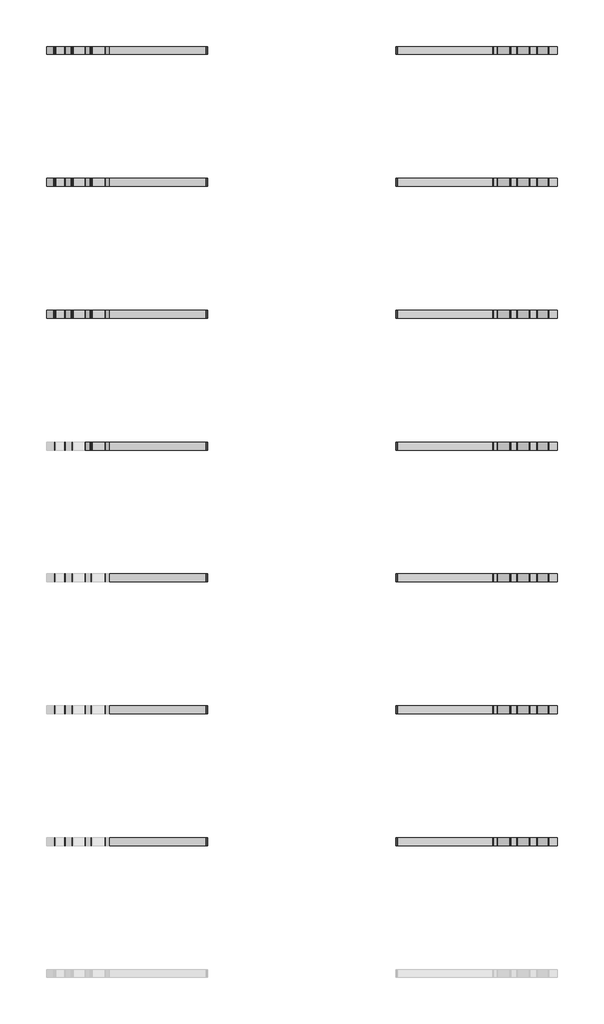
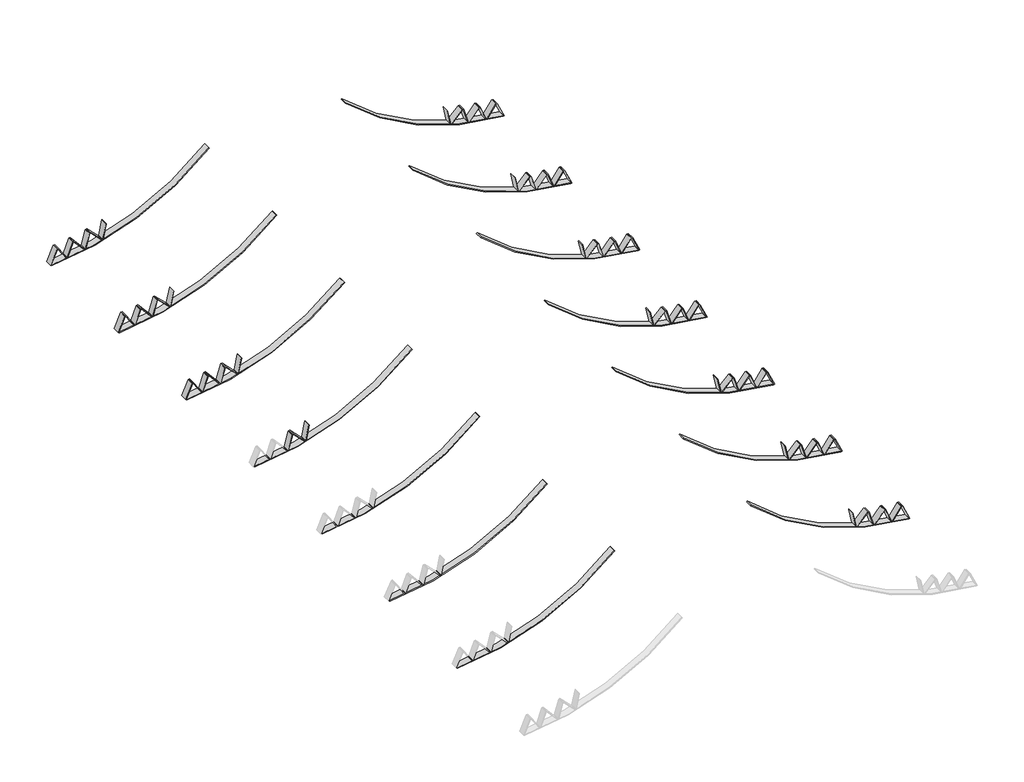
# One storey, part 4 of 4: 87 beams.
"""IFC4 building model written with IfcOpenShell, lengths in millimetres."""

import ifcopenshell
import ifcopenshell.guid

model = None  # the IFC model being written
_history = None  # IfcOwnerHistory: only IFC2X3 demands one
_inside = {}  # id of a spatial element -> (the spatial element, [elements in it])
_under = {}  # id of a project, library or spatial element -> (it, [spatial elements below it])
_declared = {}  # id of a project -> (the project, [libraries it declares])
_typed = {}  # id of a type object -> (the type object, [elements of that type])
_made_of = {}  # id of a material, layer set ... -> (it, [elements and type objects made of it])


def new_model(schema):
    """Start an empty IFC model of exactly this schema.

    Asked for "IFC4X3", IfcOpenShell would pick the latest addendum, in which some entities
    have other attributes; the version numbers below select the first issue.
    IFC2X3 requires an IfcOwnerHistory on every rooted entity: one is made here for all.
    """
    global model, _history
    if schema == "IFC4X3":
        model = ifcopenshell.file(schema_version=(4, 3, 0, 0))
    else:
        model = ifcopenshell.file(schema=schema)
    _inside.clear()
    _under.clear()
    _declared.clear()
    _typed.clear()
    _made_of.clear()
    _history = None
    if model.schema == "IFC2X3":
        org = make("IfcOrganization", Name="unknown")
        user = make(
            "IfcPersonAndOrganization",
            ThePerson=make("IfcPerson", FamilyName="unknown"),
            TheOrganization=org,
        )
        app = make(
            "IfcApplication",
            ApplicationDeveloper=org,
            Version="unknown",
            ApplicationFullName="unknown",
            ApplicationIdentifier="unknown",
        )
        _history = make(
            "IfcOwnerHistory",
            OwningUser=user,
            OwningApplication=app,
            ChangeAction="ADDED",
            CreationDate=0,
        )
    return model


def make(cls, **values):
    """One entity of the class cls with the attributes given. An attribute that is None is left unset."""
    return model.create_entity(
        cls, **{name: value for name, value in values.items() if value is not None}
    )


def rooted(cls, **values):
    """An entity with a GlobalId (a new one), such as an element, a storey or a relation."""
    return make(cls, GlobalId=ifcopenshell.guid.new(), OwnerHistory=_history, **values)


def si_unit(unit_type, name, prefix=None):
    """IfcSIUnit, for example si_unit("LENGTHUNIT", "METRE", prefix="MILLI")."""
    return make("IfcSIUnit", UnitType=unit_type, Prefix=prefix, Name=name)


def assignment(units):
    """IfcUnitAssignment: the units of a project."""
    return None if units is None else make("IfcUnitAssignment", Units=units)


def point(xyz):
    """IfcCartesianPoint."""
    return None if xyz is None else make("IfcCartesianPoint", Coordinates=xyz)


def direction(xyz):
    """IfcDirection."""
    return None if xyz is None else make("IfcDirection", DirectionRatios=xyz)


def frame(location, z_axis=None, x_axis=None):
    """IfcAxis2Placement3D, a coordinate frame: its origin and axes. An axis left out is left unset."""
    return make(
        "IfcAxis2Placement3D",
        Location=point(location),
        Axis=direction(z_axis),
        RefDirection=direction(x_axis),
    )


def frame_2d(location, x_axis=None):
    """IfcAxis2Placement2D, a coordinate frame in the plane: its origin and x axis."""
    return make(
        "IfcAxis2Placement2D", Location=point(location), RefDirection=direction(x_axis)
    )


def origin():
    """The frame at (0, 0, 0) with its axes left unset."""
    return frame((0.0, 0.0, 0.0))


def place(relative_to, where):
    """IfcLocalPlacement: puts the frame where relative to a parent placement (None: the world)."""
    return make(
        "IfcLocalPlacement", PlacementRelTo=relative_to, RelativePlacement=where
    )


def context(
    kind, dimensions, precision=None, world=None, true_north=None, identifier=None
):
    """IfcGeometricRepresentationContext, for example the 3D "Model" context."""
    return make(
        "IfcGeometricRepresentationContext",
        ContextIdentifier=identifier,
        ContextType=kind,
        CoordinateSpaceDimension=dimensions,
        Precision=precision,
        WorldCoordinateSystem=world,
        TrueNorth=true_north,
    )


def project(units=None, contexts=None):
    """IfcProject with its units and contexts."""
    return rooted(
        "IfcProject",
        Name="project",
        RepresentationContexts=contexts,
        UnitsInContext=assignment(units),
    )


def spatial(cls, under=None, at=None, **own):
    """A site, building, storey or space (cls), placed at a placement, below another one or the project."""
    s = rooted(cls, ObjectPlacement=at, **own)
    if under is not None:
        _under.setdefault(under.id(), (under, []))[1].append(s)
    return s


def polyline(points):
    """IfcPolyline through the points."""
    return make("IfcPolyline", Points=[point(p) for p in points])


def circle_curve(where, radius):
    """IfcCircle in the frame where."""
    return make("IfcCircle", Position=where, Radius=radius)


def trimmed(basis, trim1, trim2, sense, master):
    """IfcTrimmedCurve: the piece of a basis curve between two trims."""
    return make(
        "IfcTrimmedCurve",
        BasisCurve=basis,
        Trim1=trim1,
        Trim2=trim2,
        SenseAgreement=sense,
        MasterRepresentation=master,
    )


def segment(curve, same_sense, transition):
    """IfcCompositeCurveSegment."""
    return make(
        "IfcCompositeCurveSegment",
        Transition=transition,
        SameSense=same_sense,
        ParentCurve=curve,
    )


def composite_curve(segments, self_intersect=None):
    """IfcCompositeCurve: segments joined end to end."""
    return make("IfcCompositeCurve", Segments=segments, SelfIntersect=self_intersect)


def outline(outer, holes=None, kind="AREA"):
    """IfcArbitraryClosedProfileDef: a profile drawn as a closed curve; with holes, ...WithVoids."""
    if holes is None:
        return make("IfcArbitraryClosedProfileDef", ProfileType=kind, OuterCurve=outer)
    return make(
        "IfcArbitraryProfileDefWithVoids",
        ProfileType=kind,
        OuterCurve=outer,
        InnerCurves=holes,
    )


def extrude(swept, where, along, depth):
    """IfcExtrudedAreaSolid: the profile swept, set in the frame where, extruded along a direction by depth."""
    return make(
        "IfcExtrudedAreaSolid",
        SweptArea=swept,
        Position=where,
        ExtrudedDirection=direction(along),
        Depth=depth,
    )


def shape(context_of_items, identifier, shape_type, items):
    """IfcShapeRepresentation: the items that make up one representation, for example the "Body"."""
    return make(
        "IfcShapeRepresentation",
        ContextOfItems=context_of_items,
        RepresentationIdentifier=identifier,
        RepresentationType=shape_type,
        Items=items,
    )


def source(mapping_origin, context_of_items, identifier, shape_type, items):
    """IfcRepresentationMap: a shape defined once, which mapped items show again and again."""
    return make(
        "IfcRepresentationMap",
        MappingOrigin=mapping_origin,
        MappedRepresentation=shape(context_of_items, identifier, shape_type, items),
    )


def transform(
    local_origin,
    x_axis=None,
    y_axis=None,
    z_axis=None,
    scale=None,
    scale2=None,
    scale3=None,
    uniform=True,
):
    """IfcCartesianTransformationOperator3D, or its non-uniform kind. x_axis, y_axis, z_axis: its Axis1, 2, 3."""
    if uniform:
        return make(
            "IfcCartesianTransformationOperator3D",
            Axis1=direction(x_axis),
            Axis2=direction(y_axis),
            LocalOrigin=point(local_origin),
            Scale=scale,
            Axis3=direction(z_axis),
        )
    return make(
        "IfcCartesianTransformationOperator3DnonUniform",
        Axis1=direction(x_axis),
        Axis2=direction(y_axis),
        LocalOrigin=point(local_origin),
        Scale=scale,
        Axis3=direction(z_axis),
        Scale2=scale2,
        Scale3=scale3,
    )


def mapped(mapping_source, mapping_target):
    """IfcMappedItem: shows the shape of a source again, moved by a transform."""
    return make(
        "IfcMappedItem", MappingSource=mapping_source, MappingTarget=mapping_target
    )


def made_of(thing, what):
    """Note that an element or type object is made of a material, layer set ...; save() writes the relation."""
    if what is not None:
        _made_of.setdefault(what.id(), (what, []))[1].append(thing)
    return thing


def element(
    cls,
    number,
    at=None,
    inside=None,
    cuts=None,
    type_object=None,
    material=None,
    context=None,
    identifier="Body",
    shape_type=None,
    held_by="IfcProductDefinitionShape",
    body=None,
    shapes=None,
    **own,
):
    """One element of the class cls, such as IfcWall. Its Tag is "e" and its number.

    at: its placement. inside: the storey or other place that contains it. cuts: it is an
    opening in that element (IfcRelVoidsElement). A single representation is given by context,
    identifier, shape_type and body (its items); several are given by shapes. held_by: the class
    of the entity that holds the representations. save() writes the other relations.
    """
    e = rooted(cls, Tag="e%d" % number, ObjectPlacement=at, **own)
    if body is not None:
        shapes = [shape(context, identifier, shape_type, body)]
    if shapes is not None:
        e.Representation = make(held_by, Representations=shapes)
    if inside is not None:
        _inside.setdefault(inside.id(), (inside, []))[1].append(e)
    if cuts is not None:
        rooted(
            "IfcRelVoidsElement", RelatingBuildingElement=cuts, RelatedOpeningElement=e
        )
    if type_object is not None:
        _typed.setdefault(type_object.id(), (type_object, []))[1].append(e)
    return made_of(e, material)


def aggregate(whole, parts):
    """IfcRelAggregates: a whole, such as a stair, and the parts it consists of."""
    return rooted("IfcRelAggregates", RelatingObject=whole, RelatedObjects=parts)


def save(model, path):
    """Write the relations noted so far, then the file.

    IfcRelAggregates (storeys below a building ...), IfcRelContainedInSpatialStructure (elements
    in a storey), IfcRelDefinesByType, IfcRelAssociatesMaterial and IfcRelDeclares: one each for
    every whole, place, type object, material and project.
    """
    for whole, parts in _under.values():
        aggregate(whole, parts)
    for where, things in _inside.values():
        rooted(
            "IfcRelContainedInSpatialStructure",
            RelatedElements=things,
            RelatingStructure=where,
        )
    for kind, things in _typed.values():
        rooted("IfcRelDefinesByType", RelatedObjects=things, RelatingType=kind)
    for what, things in _made_of.values():
        rooted("IfcRelAssociatesMaterial", RelatedObjects=things, RelatingMaterial=what)
    for by, libraries in _declared.values():
        rooted("IfcRelDeclares", RelatingContext=by, RelatedDefinitions=libraries)
    model.write(path)


def placa_diagonal_a71479e9(model_context):
    return source(origin(), model_context, "Body", "SweptSolid", [
        extrude(outline(polyline([(161.178496, 75.0), (161.178496, -75.0), (-185.3041805, -75.0), (-185.3041805, 75.0), (161.178496, 75.0)])), frame((0.0, 0.0, -4.0), z_axis=(0.0, 0.0, 1.0), x_axis=(1.0, 0.0, 0.0)), (0.0, 0.0, 1.0), 8.0),
    ])


def placa_diagonal_67ce8334(model_context):
    return source(origin(), model_context, "Body", "SweptSolid", [
        extrude(outline(polyline([(162.9623469, 75.0), (162.9623469, -75.0), (-162.6761246, -75.0), (-162.6761246, 75.0), (162.9623469, 75.0)])), frame((0.0, 0.0, -4.0), z_axis=(0.0, 0.0, 1.0), x_axis=(1.0, 0.0, 0.0)), (0.0, 0.0, 1.0), 8.0),
    ])


def placa_diagonal_af2a04a3(model_context):
    return source(origin(), model_context, "Body", "SweptSolid", [
        extrude(outline(polyline([(165.1705216, 75.0), (165.1705216, -75.0), (-165.4962729, -75.0), (-165.4962729, 75.0), (165.1705216, 75.0)])), frame((0.0, 0.0, -4.0), z_axis=(0.0, 0.0, 1.0), x_axis=(1.0, 0.0, 0.0)), (0.0, 0.0, 1.0), 8.0),
    ])


def placa_diagonal_fb53ba7d(model_context):
    return source(origin(), model_context, "Body", "SweptSolid", [
        extrude(outline(polyline([(169.971959, 75.0), (169.971959, -75.0), (-169.5739242, -75.0), (-169.5739242, 75.0), (169.971959, 75.0)])), frame((0.0, 0.0, -4.0), z_axis=(0.0, 0.0, 1.0), x_axis=(1.0, 0.0, 0.0)), (0.0, 0.0, 1.0), 8.0),
    ])


def placa_diagonal_d1da0e1c(model_context):
    return source(origin(), model_context, "Body", "SweptSolid", [
        extrude(outline(polyline([(165.1705221, 75.0), (165.1705221, -75.0), (-165.4962734, -75.0), (-165.4962734, 75.0), (165.1705221, 75.0)])), frame((0.0, 0.0, -4.0), z_axis=(0.0, 0.0, 1.0), x_axis=(1.0, 0.0, 0.0)), (0.0, 0.0, 1.0), 8.0),
    ])


def placa_diagonal_6d03bdc5(model_context):
    return source(origin(), model_context, "Body", "SweptSolid", [
        extrude(outline(polyline([(191.209825, 75.0), (191.209825, -75.0), (-166.9394885, -75.0), (-166.9394885, 75.0), (191.209825, 75.0)])), frame((0.0, 0.0, -4.0), z_axis=(0.0, 0.0, 1.0), x_axis=(1.0, 0.0, 0.0)), (0.0, 0.0, 1.0), 8.0),
    ])


def placa_diagonal_30fa4039(model_context):
    return source(origin(), model_context, "Body", "SweptSolid", [
        extrude(outline(polyline([(167.0675386, 75.0), (167.0675386, -75.0), (-167.4240159, -75.0), (-167.4240159, 75.0), (167.0675386, 75.0)])), frame((0.0, 0.0, -4.0), z_axis=(0.0, 0.0, 1.0), x_axis=(1.0, 0.0, 0.0)), (0.0, 0.0, 1.0), 8.0),
    ])


def placa_diagonal_ded414cc(model_context):
    return source(origin(), model_context, "Body", "SweptSolid", [
        extrude(outline(polyline([(167.4240165, 75.0), (167.4240165, -75.0), (-167.0675392, -75.0), (-167.0675392, 75.0), (167.4240165, 75.0)])), frame((0.0, 0.0, -4.0), z_axis=(0.0, 0.0, 1.0), x_axis=(1.0, 0.0, 0.0)), (0.0, 0.0, 1.0), 8.0),
    ])


def placa_diagonal_4690b74a(model_context):
    return source(origin(), model_context, "Body", "SweptSolid", [
        extrude(outline(polyline([(167.0675389, 75.0), (167.0675389, -75.0), (-167.4240162, -75.0), (-167.4240162, 75.0), (167.0675389, 75.0)])), frame((0.0, 0.0, -4.0), z_axis=(0.0, 0.0, 1.0), x_axis=(1.0, 0.0, 0.0)), (0.0, 0.0, 1.0), 8.0),
    ])


def placa_diagonal_aaf0c3b6(model_context):
    return source(origin(), model_context, "Body", "SweptSolid", [
        extrude(outline(polyline([(167.4240163, 75.0), (167.4240163, -75.0), (-167.067539, -75.0), (-167.067539, 75.0), (167.4240163, 75.0)])), frame((0.0, 0.0, -4.0), z_axis=(0.0, 0.0, 1.0), x_axis=(1.0, 0.0, 0.0)), (0.0, 0.0, 1.0), 8.0),
    ])


model = new_model("IFC4")

# Units and contexts
model_context = context("Model", 3, world=origin())
ifc_project = project(units=[si_unit("LENGTHUNIT", "METRE", prefix="MILLI")], contexts=[model_context])

# Site, building, storey
site = spatial("IfcSite", under=ifc_project)
building = spatial("IfcBuilding", under=site)
storey = spatial("IfcBuildingStorey", under=building, Name="Nível 4", Elevation=48165.0)

# Beams
placement = place(None, origin())
element("IfcBeam", 1, ObjectType="Placa : banzo", at=placement, inside=storey, context=model_context, shape_type="SweptSolid", body=[
    extrude(outline(composite_curve([segment(polyline([(48158.5516223, 8114.9704041), (48174.5198715, 8115.9778843)]), True, "CONTINUOUS"), segment(trimmed(circle_curve(frame_2d((53506.1312788, 8452.3636953)), 5342.2126139), [point((48174.5198715, 8115.9778843))], [point((49646.1683419, 4759.1372282))], True, "CARTESIAN"), True, "CONTINUOUS"), segment(polyline([(49646.1683419, 4759.1372282), (49634.6077, 4748.0759643)]), True, "CONTINUOUS"), segment(trimmed(circle_curve(frame_2d((53506.1312788, 8452.3636953)), 5358.2126139), [point((49634.6077, 4748.0759643))], [point((48158.5516223, 8114.9704041))], False, "CARTESIAN"), True, "CONTINUOUS")], self_intersect=False)), frame((0.0, 15321.4376366, 0.0), z_axis=(0.0, 1.0, 0.0), x_axis=(0.0, 0.0, 1.0)), (0.0, 0.0, 1.0), 150.0),
])
element("IfcBeam", 2, ObjectType="Placa : banzo", at=placement, inside=storey, context=model_context, shape_type="SweptSolid", body=[
    extrude(outline(composite_curve([segment(polyline([(49634.6077, 1843.8240278), (49646.1683419, 1832.762764)]), True, "CONTINUOUS"), segment(trimmed(circle_curve(frame_2d((53506.1312788, -1860.4637031)), 5342.2126139), [point((49646.1683419, 1832.762764))], [point((48174.5198715, -1524.0778921))], True, "CARTESIAN"), True, "CONTINUOUS"), segment(polyline([(48174.5198715, -1524.0778921), (48158.5516223, -1523.070412)]), True, "CONTINUOUS"), segment(trimmed(circle_curve(frame_2d((53506.1312788, -1860.4637031)), 5358.2126139), [point((48158.5516223, -1523.070412))], [point((49634.6077, 1843.8240278))], False, "CARTESIAN"), True, "CONTINUOUS")], self_intersect=False)), frame((0.0, 15321.4376366, 0.0), z_axis=(0.0, 1.0, 0.0), x_axis=(0.0, 0.0, 1.0)), (0.0, 0.0, 1.0), 150.0),
])
element("IfcBeam", 3, ObjectType="Placa : banzo", at=placement, inside=storey, context=model_context, shape_type="SweptSolid", body=[
    extrude(outline(composite_curve([segment(polyline([(48158.5516223, 8114.9704041), (48174.5198715, 8115.9778843)]), True, "CONTINUOUS"), segment(trimmed(circle_curve(frame_2d((53506.1312788, 8452.3636953)), 5342.2126139), [point((48174.5198715, 8115.9778843))], [point((49646.1683419, 4759.1372282))], True, "CARTESIAN"), True, "CONTINUOUS"), segment(polyline([(49646.1683419, 4759.1372282), (49634.6077, 4748.0759643)]), True, "CONTINUOUS"), segment(trimmed(circle_curve(frame_2d((53506.1312788, 8452.3636953)), 5358.2126139), [point((49634.6077, 4748.0759643))], [point((48158.5516223, 8114.9704041))], False, "CARTESIAN"), True, "CONTINUOUS")], self_intersect=False)), frame((0.0, 12821.4376366, 0.0), z_axis=(0.0, 1.0, 0.0), x_axis=(0.0, 0.0, 1.0)), (0.0, 0.0, 1.0), 150.0),
])
element("IfcBeam", 4, ObjectType="Placa : banzo", at=placement, inside=storey, context=model_context, shape_type="SweptSolid", body=[
    extrude(outline(composite_curve([segment(polyline([(49634.6077, 1843.8240278), (49646.1683419, 1832.762764)]), True, "CONTINUOUS"), segment(trimmed(circle_curve(frame_2d((53506.1312788, -1860.4637031)), 5342.2126139), [point((49646.1683419, 1832.762764))], [point((48174.5198715, -1524.0778921))], True, "CARTESIAN"), True, "CONTINUOUS"), segment(polyline([(48174.5198715, -1524.0778921), (48158.5516223, -1523.070412)]), True, "CONTINUOUS"), segment(trimmed(circle_curve(frame_2d((53506.1312788, -1860.4637031)), 5358.2126139), [point((48158.5516223, -1523.070412))], [point((49634.6077, 1843.8240278))], False, "CARTESIAN"), True, "CONTINUOUS")], self_intersect=False)), frame((0.0, 12821.4376366, 0.0), z_axis=(0.0, 1.0, 0.0), x_axis=(0.0, 0.0, 1.0)), (0.0, 0.0, 1.0), 150.0),
])
element("IfcBeam", 5, ObjectType="Placa : banzo", at=placement, inside=storey, context=model_context, shape_type="SweptSolid", body=[
    extrude(outline(composite_curve([segment(polyline([(48158.5516223, 8114.9704041), (48174.5198715, 8115.9778843)]), True, "CONTINUOUS"), segment(trimmed(circle_curve(frame_2d((53506.1312788, 8452.3636953)), 5342.2126139), [point((48174.5198715, 8115.9778843))], [point((49646.1683419, 4759.1372282))], True, "CARTESIAN"), True, "CONTINUOUS"), segment(polyline([(49646.1683419, 4759.1372282), (49634.6077, 4748.0759643)]), True, "CONTINUOUS"), segment(trimmed(circle_curve(frame_2d((53506.1312788, 8452.3636953)), 5358.2126139), [point((49634.6077, 4748.0759643))], [point((48158.5516223, 8114.9704041))], False, "CARTESIAN"), True, "CONTINUOUS")], self_intersect=False)), frame((0.0, 10321.4376366, 0.0), z_axis=(0.0, 1.0, 0.0), x_axis=(0.0, 0.0, 1.0)), (0.0, 0.0, 1.0), 150.0),
])
element("IfcBeam", 6, ObjectType="Placa : banzo", at=placement, inside=storey, context=model_context, shape_type="SweptSolid", body=[
    extrude(outline(composite_curve([segment(polyline([(49634.6077, 1843.8240278), (49646.1683419, 1832.762764)]), True, "CONTINUOUS"), segment(trimmed(circle_curve(frame_2d((53506.1312788, -1860.4637031)), 5342.2126139), [point((49646.1683419, 1832.762764))], [point((48174.5198715, -1524.0778921))], True, "CARTESIAN"), True, "CONTINUOUS"), segment(polyline([(48174.5198715, -1524.0778921), (48158.5516223, -1523.070412)]), True, "CONTINUOUS"), segment(trimmed(circle_curve(frame_2d((53506.1312788, -1860.4637031)), 5358.2126139), [point((48158.5516223, -1523.070412))], [point((49634.6077, 1843.8240278))], False, "CARTESIAN"), True, "CONTINUOUS")], self_intersect=False)), frame((0.0, 10321.4376366, 0.0), z_axis=(0.0, 1.0, 0.0), x_axis=(0.0, 0.0, 1.0)), (0.0, 0.0, 1.0), 150.0),
])
element("IfcBeam", 7, ObjectType="Placa : banzo", at=placement, inside=storey, context=model_context, shape_type="SweptSolid", body=[
    extrude(outline(composite_curve([segment(polyline([(48158.5516223, 8114.9704041), (48174.5198715, 8115.9778843)]), True, "CONTINUOUS"), segment(trimmed(circle_curve(frame_2d((53506.1312788, 8452.3636953)), 5342.2126139), [point((48174.5198715, 8115.9778843))], [point((49646.1683419, 4759.1372282))], True, "CARTESIAN"), True, "CONTINUOUS"), segment(polyline([(49646.1683419, 4759.1372282), (49634.6077, 4748.0759643)]), True, "CONTINUOUS"), segment(trimmed(circle_curve(frame_2d((53506.1312788, 8452.3636953)), 5358.2126139), [point((49634.6077, 4748.0759643))], [point((48158.5516223, 8114.9704041))], False, "CARTESIAN"), True, "CONTINUOUS")], self_intersect=False)), frame((0.0, 7821.4376366, 0.0), z_axis=(0.0, 1.0, 0.0), x_axis=(0.0, 0.0, 1.0)), (0.0, 0.0, 1.0), 150.0),
])
element("IfcBeam", 8, ObjectType="Placa : banzo", at=placement, inside=storey, context=model_context, shape_type="SweptSolid", body=[
    extrude(outline(composite_curve([segment(polyline([(49634.6077, 1843.8240278), (49646.1683419, 1832.762764)]), True, "CONTINUOUS"), segment(trimmed(circle_curve(frame_2d((53506.1312788, -1860.4637031)), 5342.2126139), [point((49646.1683419, 1832.762764))], [point((48174.5198715, -1524.0778921))], True, "CARTESIAN"), True, "CONTINUOUS"), segment(polyline([(48174.5198715, -1524.0778921), (48158.5516223, -1523.070412)]), True, "CONTINUOUS"), segment(trimmed(circle_curve(frame_2d((53506.1312788, -1860.4637031)), 5358.2126139), [point((48158.5516223, -1523.070412))], [point((49634.6077, 1843.8240278))], False, "CARTESIAN"), True, "CONTINUOUS")], self_intersect=False)), frame((0.0, 7821.4376366, 0.0), z_axis=(0.0, 1.0, 0.0), x_axis=(0.0, 0.0, 1.0)), (0.0, 0.0, 1.0), 150.0),
])
element("IfcBeam", 9, ObjectType="Placa : banzo", at=placement, inside=storey, context=model_context, shape_type="SweptSolid", body=[
    extrude(outline(composite_curve([segment(polyline([(48158.5516223, 8114.9704041), (48174.5198715, 8115.9778843)]), True, "CONTINUOUS"), segment(trimmed(circle_curve(frame_2d((53506.1312788, 8452.3636953)), 5342.2126139), [point((48174.5198715, 8115.9778843))], [point((49646.1683419, 4759.1372282))], True, "CARTESIAN"), True, "CONTINUOUS"), segment(polyline([(49646.1683419, 4759.1372282), (49634.6077, 4748.0759643)]), True, "CONTINUOUS"), segment(trimmed(circle_curve(frame_2d((53506.1312788, 8452.3636953)), 5358.2126139), [point((49634.6077, 4748.0759643))], [point((48158.5516223, 8114.9704041))], False, "CARTESIAN"), True, "CONTINUOUS")], self_intersect=False)), frame((0.0, 5321.4376366, 0.0), z_axis=(0.0, 1.0, 0.0), x_axis=(0.0, 0.0, 1.0)), (0.0, 0.0, 1.0), 150.0),
])
element("IfcBeam", 10, ObjectType="Placa : banzo", at=placement, inside=storey, context=model_context, shape_type="SweptSolid", body=[
    extrude(outline(composite_curve([segment(polyline([(49634.6077, 1843.8240278), (49646.1683419, 1832.762764)]), True, "CONTINUOUS"), segment(trimmed(circle_curve(frame_2d((53506.1312788, -1860.4637031)), 5342.2126139), [point((49646.1683419, 1832.762764))], [point((48174.5198715, -1524.0778921))], True, "CARTESIAN"), True, "CONTINUOUS"), segment(polyline([(48174.5198715, -1524.0778921), (48158.5516223, -1523.070412)]), True, "CONTINUOUS"), segment(trimmed(circle_curve(frame_2d((53506.1312788, -1860.4637031)), 5358.2126139), [point((48158.5516223, -1523.070412))], [point((49634.6077, 1843.8240278))], False, "CARTESIAN"), True, "CONTINUOUS")], self_intersect=False)), frame((0.0, 5321.4376366, 0.0), z_axis=(0.0, 1.0, 0.0), x_axis=(0.0, 0.0, 1.0)), (0.0, 0.0, 1.0), 150.0),
])
element("IfcBeam", 11, ObjectType="Placa : banzo", at=placement, inside=storey, context=model_context, shape_type="SweptSolid", body=[
    extrude(outline(composite_curve([segment(polyline([(48158.5516223, 8114.9704041), (48174.5198715, 8115.9778843)]), True, "CONTINUOUS"), segment(trimmed(circle_curve(frame_2d((53506.1312788, 8452.3636953)), 5342.2126139), [point((48174.5198715, 8115.9778843))], [point((49646.1683419, 4759.1372282))], True, "CARTESIAN"), True, "CONTINUOUS"), segment(polyline([(49646.1683419, 4759.1372282), (49634.6077, 4748.0759643)]), True, "CONTINUOUS"), segment(trimmed(circle_curve(frame_2d((53506.1312788, 8452.3636953)), 5358.2126139), [point((49634.6077, 4748.0759643))], [point((48158.5516223, 8114.9704041))], False, "CARTESIAN"), True, "CONTINUOUS")], self_intersect=False)), frame((0.0, 2821.4376366, 0.0), z_axis=(0.0, 1.0, 0.0), x_axis=(0.0, 0.0, 1.0)), (0.0, 0.0, 1.0), 150.0),
])
element("IfcBeam", 12, ObjectType="Placa : banzo", at=placement, inside=storey, context=model_context, shape_type="SweptSolid", body=[
    extrude(outline(composite_curve([segment(polyline([(49634.6077, 1843.8240278), (49646.1683419, 1832.762764)]), True, "CONTINUOUS"), segment(trimmed(circle_curve(frame_2d((53506.1312788, -1860.4637031)), 5342.2126139), [point((49646.1683419, 1832.762764))], [point((48174.5198715, -1524.0778921))], True, "CARTESIAN"), True, "CONTINUOUS"), segment(polyline([(48174.5198715, -1524.0778921), (48158.5516223, -1523.070412)]), True, "CONTINUOUS"), segment(trimmed(circle_curve(frame_2d((53506.1312788, -1860.4637031)), 5358.2126139), [point((48158.5516223, -1523.070412))], [point((49634.6077, 1843.8240278))], False, "CARTESIAN"), True, "CONTINUOUS")], self_intersect=False)), frame((0.0, 2821.4376366, 0.0), z_axis=(0.0, 1.0, 0.0), x_axis=(0.0, 0.0, 1.0)), (0.0, 0.0, 1.0), 150.0),
])
element("IfcBeam", 13, ObjectType="Placa : banzo", at=placement, inside=storey, context=model_context, shape_type="SweptSolid", body=[
    extrude(outline(composite_curve([segment(polyline([(48158.5516223, 8114.9704041), (48174.5198715, 8115.9778843)]), True, "CONTINUOUS"), segment(trimmed(circle_curve(frame_2d((53506.1312788, 8452.3636953)), 5342.2126139), [point((48174.5198715, 8115.9778843))], [point((49646.1683419, 4759.1372282))], True, "CARTESIAN"), True, "CONTINUOUS"), segment(polyline([(49646.1683419, 4759.1372282), (49634.6077, 4748.0759643)]), True, "CONTINUOUS"), segment(trimmed(circle_curve(frame_2d((53506.1312788, 8452.3636953)), 5358.2126139), [point((49634.6077, 4748.0759643))], [point((48158.5516223, 8114.9704041))], False, "CARTESIAN"), True, "CONTINUOUS")], self_intersect=False)), frame((0.0, 321.4376366, 0.0), z_axis=(0.0, 1.0, 0.0), x_axis=(0.0, 0.0, 1.0)), (0.0, 0.0, 1.0), 150.0),
])
element("IfcBeam", 14, ObjectType="Placa : banzo", at=placement, inside=storey, context=model_context, shape_type="SweptSolid", body=[
    extrude(outline(composite_curve([segment(polyline([(49634.6077, 1843.8240278), (49646.1683419, 1832.762764)]), True, "CONTINUOUS"), segment(trimmed(circle_curve(frame_2d((53506.1312788, -1860.4637031)), 5342.2126139), [point((49646.1683419, 1832.762764))], [point((48174.5198715, -1524.0778921))], True, "CARTESIAN"), True, "CONTINUOUS"), segment(polyline([(48174.5198715, -1524.0778921), (48158.5516223, -1523.070412)]), True, "CONTINUOUS"), segment(trimmed(circle_curve(frame_2d((53506.1312788, -1860.4637031)), 5358.2126139), [point((48158.5516223, -1523.070412))], [point((49634.6077, 1843.8240278))], False, "CARTESIAN"), True, "CONTINUOUS")], self_intersect=False)), frame((0.0, 321.4376366, 0.0), z_axis=(0.0, 1.0, 0.0), x_axis=(0.0, 0.0, 1.0)), (0.0, 0.0, 1.0), 150.0),
])
placa_diagonal_shape = placa_diagonal_a71479e9(model_context)
element("IfcBeam", 15, ObjectType="Placa : diagonal", at=placement, inside=storey, context=model_context, shape_type="MappedRepresentation", body=[
    mapped(placa_diagonal_shape, transform((-1468.5029422, 15396.4376366, 48342.5238752), x_axis=(0.4074605623535313, 0.0, 0.9132228042085588), y_axis=(0.0, -1.0, 0.0), z_axis=(0.9132228042085588, 0.0, -0.4074605623535313))),
])
element("IfcBeam", 16, ObjectType="Placa : diagonal", at=placement, inside=storey, context=model_context, shape_type="MappedRepresentation", body=[
    mapped(placa_diagonal_shape, transform((-1468.5029422, 12896.4376366, 48342.5238752), x_axis=(0.4074605623535313, 0.0, 0.9132228042085588), y_axis=(0.0, -1.0, 0.0), z_axis=(0.9132228042085588, 0.0, -0.4074605623535313))),
])
element("IfcBeam", 17, ObjectType="Placa : diagonal", at=placement, inside=storey, context=model_context, shape_type="MappedRepresentation", body=[
    mapped(placa_diagonal_shape, transform((-1468.5029422, 10396.4376366, 48342.5238752), x_axis=(0.4074605623535313, 0.0, 0.9132228042085588), y_axis=(0.0, -1.0, 0.0), z_axis=(0.9132228042085588, 0.0, -0.4074605623535313))),
])
placa_diagonal_2_shape = placa_diagonal_67ce8334(model_context)
element("IfcBeam", 18, ObjectType="Placa : diagonal", at=placement, inside=storey, context=model_context, shape_type="MappedRepresentation", body=[
    mapped(placa_diagonal_2_shape, transform((-1292.3410904, 15396.4376366, 48354.815057), x_axis=(0.5398932132172984, 0.0, -0.8417335197803998), y_axis=(0.0, -1.0, 0.0), z_axis=(-0.8417335197803998, 0.0, -0.5398932132172984))),
])
element("IfcBeam", 19, ObjectType="Placa : diagonal", at=placement, inside=storey, context=model_context, shape_type="MappedRepresentation", body=[
    mapped(placa_diagonal_2_shape, transform((-1292.3410904, 12896.4376366, 48354.815057), x_axis=(0.5398932132172984, 0.0, -0.8417335197803998), y_axis=(0.0, -1.0, 0.0), z_axis=(-0.8417335197803998, 0.0, -0.5398932132172984))),
])
element("IfcBeam", 20, ObjectType="Placa : diagonal", at=placement, inside=storey, context=model_context, shape_type="MappedRepresentation", body=[
    mapped(placa_diagonal_2_shape, transform((-1292.3410904, 10396.4376366, 48354.815057), x_axis=(0.5398932132172984, 0.0, -0.8417335197803998), y_axis=(0.0, -1.0, 0.0), z_axis=(-0.8417335197803998, 0.0, -0.5398932132172984))),
])
placa_diagonal_3_shape = placa_diagonal_af2a04a3(model_context)
element("IfcBeam", 21, ObjectType="Placa : diagonal", at=placement, inside=storey, context=model_context, shape_type="MappedRepresentation", body=[
    mapped(placa_diagonal_3_shape, transform((-1127.2550828, 15396.4376366, 48375.8118772), x_axis=(0.3404667803509138, 0.0, 0.940256545564817), y_axis=(0.0, -1.0, 0.0), z_axis=(0.940256545564817, 0.0, -0.3404667803509138))),
])
element("IfcBeam", 22, ObjectType="Placa : diagonal", at=placement, inside=storey, context=model_context, shape_type="MappedRepresentation", body=[
    mapped(placa_diagonal_3_shape, transform((-392.7303205, 15396.4376366, 48535.8666224), x_axis=(0.20085127706480188, 0.0, 0.9796217456250337), y_axis=(0.0, -1.0, 0.0), z_axis=(0.9796217456250337, 0.0, -0.20085127706480188))),
])
element("IfcBeam", 23, ObjectType="Placa : diagonal", at=placement, inside=storey, context=model_context, shape_type="MappedRepresentation", body=[
    mapped(placa_diagonal_3_shape, transform((-1127.2550828, 12896.4376366, 48375.8118772), x_axis=(0.3404667803509138, 0.0, 0.940256545564817), y_axis=(0.0, -1.0, 0.0), z_axis=(0.940256545564817, 0.0, -0.3404667803509138))),
])
element("IfcBeam", 24, ObjectType="Placa : diagonal", at=placement, inside=storey, context=model_context, shape_type="MappedRepresentation", body=[
    mapped(placa_diagonal_3_shape, transform((-392.7303205, 12896.4376366, 48535.8666224), x_axis=(0.20085127706480188, 0.0, 0.9796217456250337), y_axis=(0.0, -1.0, 0.0), z_axis=(0.9796217456250337, 0.0, -0.20085127706480188))),
])
element("IfcBeam", 25, ObjectType="Placa : diagonal", at=placement, inside=storey, context=model_context, shape_type="MappedRepresentation", body=[
    mapped(placa_diagonal_3_shape, transform((-1127.2550828, 10396.4376366, 48375.8118772), x_axis=(0.3404667803509138, 0.0, 0.940256545564817), y_axis=(0.0, -1.0, 0.0), z_axis=(0.940256545564817, 0.0, -0.3404667803509138))),
])
element("IfcBeam", 26, ObjectType="Placa : diagonal", at=placement, inside=storey, context=model_context, shape_type="MappedRepresentation", body=[
    mapped(placa_diagonal_3_shape, transform((-392.7303205, 10396.4376366, 48535.8666224), x_axis=(0.20085127706480188, 0.0, 0.9796217456250337), y_axis=(0.0, -1.0, 0.0), z_axis=(0.9796217456250337, 0.0, -0.20085127706480188))),
])
element("IfcBeam", 27, ObjectType="Placa : diagonal", at=placement, inside=storey, context=model_context, shape_type="MappedRepresentation", body=[
    mapped(placa_diagonal_3_shape, transform((-392.7303205, 7896.4376366, 48535.8666224), x_axis=(0.20085127706480188, 0.0, 0.9796217456250337), y_axis=(0.0, -1.0, 0.0), z_axis=(0.9796217456250337, 0.0, -0.20085127706480188))),
])
placa_diagonal_4_shape = placa_diagonal_fb53ba7d(model_context)
element("IfcBeam", 28, ObjectType="Placa : diagonal", at=placement, inside=storey, context=model_context, shape_type="MappedRepresentation", body=[
    mapped(placa_diagonal_4_shape, transform((-935.6334765, 15396.4376366, 48407.0552778), x_axis=(0.6551223780870831, 0.0, -0.7555227790937377), y_axis=(0.0, -1.0, 0.0), z_axis=(-0.7555227790937377, 0.0, -0.6551223780870831))),
])
element("IfcBeam", 29, ObjectType="Placa : diagonal", at=placement, inside=storey, context=model_context, shape_type="MappedRepresentation", body=[
    mapped(placa_diagonal_4_shape, transform((-568.2358431, 15396.4376366, 48487.5623421), x_axis=(0.7081946416059488, 0.0, -0.706017244549042), y_axis=(0.0, -1.0, 0.0), z_axis=(-0.706017244549042, 0.0, -0.7081946416059488))),
])
element("IfcBeam", 30, ObjectType="Placa : diagonal", at=placement, inside=storey, context=model_context, shape_type="MappedRepresentation", body=[
    mapped(placa_diagonal_4_shape, transform((-935.6334765, 12896.4376366, 48407.0552778), x_axis=(0.6551223780870831, 0.0, -0.7555227790937377), y_axis=(0.0, -1.0, 0.0), z_axis=(-0.7555227790937377, 0.0, -0.6551223780870831))),
])
element("IfcBeam", 31, ObjectType="Placa : diagonal", at=placement, inside=storey, context=model_context, shape_type="MappedRepresentation", body=[
    mapped(placa_diagonal_4_shape, transform((-568.2358431, 12896.4376366, 48487.5623421), x_axis=(0.7081946416059488, 0.0, -0.706017244549042), y_axis=(0.0, -1.0, 0.0), z_axis=(-0.706017244549042, 0.0, -0.7081946416059488))),
])
element("IfcBeam", 32, ObjectType="Placa : diagonal", at=placement, inside=storey, context=model_context, shape_type="MappedRepresentation", body=[
    mapped(placa_diagonal_4_shape, transform((-935.6334765, 10396.4376366, 48407.0552778), x_axis=(0.6551223780870831, 0.0, -0.7555227790937377), y_axis=(0.0, -1.0, 0.0), z_axis=(-0.7555227790937377, 0.0, -0.6551223780870831))),
])
element("IfcBeam", 33, ObjectType="Placa : diagonal", at=placement, inside=storey, context=model_context, shape_type="MappedRepresentation", body=[
    mapped(placa_diagonal_4_shape, transform((-568.2358431, 10396.4376366, 48487.5623421), x_axis=(0.7081946416059488, 0.0, -0.706017244549042), y_axis=(0.0, -1.0, 0.0), z_axis=(-0.706017244549042, 0.0, -0.7081946416059488))),
])
element("IfcBeam", 34, ObjectType="Placa : diagonal", at=placement, inside=storey, context=model_context, shape_type="MappedRepresentation", body=[
    mapped(placa_diagonal_4_shape, transform((-568.2358431, 7896.4376366, 48487.5623421), x_axis=(0.7081946416059488, 0.0, -0.706017244549042), y_axis=(0.0, -1.0, 0.0), z_axis=(-0.706017244549042, 0.0, -0.7081946416059488))),
])
placa_diagonal_5_shape = placa_diagonal_d1da0e1c(model_context)
element("IfcBeam", 35, ObjectType="Placa : diagonal", at=placement, inside=storey, context=model_context, shape_type="MappedRepresentation", body=[
    mapped(placa_diagonal_5_shape, transform((-757.0867023, 15396.4376366, 48442.5030113), x_axis=(0.2713737594345945, 0.0, 0.9624740426059993), y_axis=(0.0, -1.0, 0.0), z_axis=(0.9624740426059993, 0.0, -0.2713737594345945))),
])
element("IfcBeam", 36, ObjectType="Placa : diagonal", at=placement, inside=storey, context=model_context, shape_type="MappedRepresentation", body=[
    mapped(placa_diagonal_5_shape, transform((-757.0867023, 12896.4376366, 48442.5030113), x_axis=(0.2713737594345945, 0.0, 0.9624740426059993), y_axis=(0.0, -1.0, 0.0), z_axis=(0.9624740426059993, 0.0, -0.2713737594345945))),
])
element("IfcBeam", 37, ObjectType="Placa : diagonal", at=placement, inside=storey, context=model_context, shape_type="MappedRepresentation", body=[
    mapped(placa_diagonal_5_shape, transform((-757.0867023, 10396.4376366, 48442.5030113), x_axis=(0.2713737594345945, 0.0, 0.9624740426059993), y_axis=(0.0, -1.0, 0.0), z_axis=(0.9624740426059993, 0.0, -0.2713737594345945))),
])
element("IfcBeam", 38, ObjectType="Placa : diagonal", at=placement, inside=storey, context=model_context, shape_type="MappedRepresentation", body=[
    mapped(placa_diagonal_5_shape, transform((-757.0867023, 7896.4376366, 48442.5030113), x_axis=(0.2713737594345945, 0.0, 0.9624740426059993), y_axis=(0.0, -1.0, 0.0), z_axis=(0.9624740426059993, 0.0, -0.2713737594345945))),
])
placa_diagonal_6_shape = placa_diagonal_6d03bdc5(model_context)
element("IfcBeam", 39, ObjectType="Placa : diagonal", at=placement, inside=storey, context=model_context, shape_type="MappedRepresentation", body=[
    mapped(placa_diagonal_6_shape, transform((8059.7198757, 15396.4376366, 48338.6280973), x_axis=(0.4189773842608123, 0.0, -0.9079966693099526), y_axis=(0.0, -1.0, 0.0), z_axis=(-0.9079966693099526, 0.0, -0.4189773842608123))),
])
element("IfcBeam", 40, ObjectType="Placa : diagonal", at=placement, inside=storey, context=model_context, shape_type="MappedRepresentation", body=[
    mapped(placa_diagonal_6_shape, transform((8059.7198757, 12896.4376366, 48338.6280973), x_axis=(0.4189773842608123, 0.0, -0.9079966693099526), y_axis=(0.0, -1.0, 0.0), z_axis=(-0.9079966693099526, 0.0, -0.4189773842608123))),
])
element("IfcBeam", 41, ObjectType="Placa : diagonal", at=placement, inside=storey, context=model_context, shape_type="MappedRepresentation", body=[
    mapped(placa_diagonal_6_shape, transform((8059.7198757, 10396.4376366, 48338.6280973), x_axis=(0.4189773842608123, 0.0, -0.9079966693099526), y_axis=(0.0, -1.0, 0.0), z_axis=(-0.9079966693099526, 0.0, -0.4189773842608123))),
])
element("IfcBeam", 42, ObjectType="Placa : diagonal", at=placement, inside=storey, context=model_context, shape_type="MappedRepresentation", body=[
    mapped(placa_diagonal_6_shape, transform((8059.7198757, 7896.4376366, 48338.6280973), x_axis=(0.4189773842608123, 0.0, -0.9079966693099526), y_axis=(0.0, -1.0, 0.0), z_axis=(-0.9079966693099526, 0.0, -0.4189773842608123))),
])
element("IfcBeam", 43, ObjectType="Placa : diagonal", at=placement, inside=storey, context=model_context, shape_type="MappedRepresentation", body=[
    mapped(placa_diagonal_6_shape, transform((8059.7198757, 5396.4376366, 48338.6280973), x_axis=(0.4189773842608123, 0.0, -0.9079966693099526), y_axis=(0.0, -1.0, 0.0), z_axis=(-0.9079966693099526, 0.0, -0.4189773842608123))),
])
element("IfcBeam", 44, ObjectType="Placa : diagonal", at=placement, inside=storey, context=model_context, shape_type="MappedRepresentation", body=[
    mapped(placa_diagonal_6_shape, transform((8059.7198757, 2896.4376366, 48338.6280973), x_axis=(0.4189773842608123, 0.0, -0.9079966693099526), y_axis=(0.0, -1.0, 0.0), z_axis=(-0.9079966693099526, 0.0, -0.4189773842608123))),
])
element("IfcBeam", 45, ObjectType="Placa : diagonal", at=placement, inside=storey, context=model_context, shape_type="MappedRepresentation", body=[
    mapped(placa_diagonal_6_shape, transform((8059.7198757, 396.4376366, 48338.6280973), x_axis=(0.4189773842608123, 0.0, -0.9079966693099526), y_axis=(0.0, -1.0, 0.0), z_axis=(-0.9079966693099526, 0.0, -0.4189773842608123))),
])
placa_diagonal_7_shape = placa_diagonal_30fa4039(model_context)
element("IfcBeam", 46, ObjectType="Placa : diagonal", at=placement, inside=storey, context=model_context, shape_type="MappedRepresentation", body=[
    mapped(placa_diagonal_7_shape, transform((7867.9931921, 15396.4376366, 48356.8132581), x_axis=(0.5832804616623758, 0.0, 0.8122708310920229), y_axis=(0.0, -1.0, 0.0), z_axis=(0.8122708310920229, 0.0, -0.5832804616623758))),
])
element("IfcBeam", 47, ObjectType="Placa : diagonal", at=placement, inside=storey, context=model_context, shape_type="MappedRepresentation", body=[
    mapped(placa_diagonal_7_shape, transform((7867.9931921, 12896.4376366, 48356.8132581), x_axis=(0.5832804616623758, 0.0, 0.8122708310920229), y_axis=(0.0, -1.0, 0.0), z_axis=(0.8122708310920229, 0.0, -0.5832804616623758))),
])
element("IfcBeam", 48, ObjectType="Placa : diagonal", at=placement, inside=storey, context=model_context, shape_type="MappedRepresentation", body=[
    mapped(placa_diagonal_7_shape, transform((7867.9931921, 10396.4376366, 48356.8132581), x_axis=(0.5832804616623758, 0.0, 0.8122708310920229), y_axis=(0.0, -1.0, 0.0), z_axis=(0.8122708310920229, 0.0, -0.5832804616623758))),
])
element("IfcBeam", 49, ObjectType="Placa : diagonal", at=placement, inside=storey, context=model_context, shape_type="MappedRepresentation", body=[
    mapped(placa_diagonal_7_shape, transform((7867.9931921, 7896.4376366, 48356.8132581), x_axis=(0.5832804616623758, 0.0, 0.8122708310920229), y_axis=(0.0, -1.0, 0.0), z_axis=(0.8122708310920229, 0.0, -0.5832804616623758))),
])
element("IfcBeam", 50, ObjectType="Placa : diagonal", at=placement, inside=storey, context=model_context, shape_type="MappedRepresentation", body=[
    mapped(placa_diagonal_7_shape, transform((7867.9931921, 5396.4376366, 48356.8132581), x_axis=(0.5832804616623758, 0.0, 0.8122708310920229), y_axis=(0.0, -1.0, 0.0), z_axis=(0.8122708310920229, 0.0, -0.5832804616623758))),
])
element("IfcBeam", 51, ObjectType="Placa : diagonal", at=placement, inside=storey, context=model_context, shape_type="MappedRepresentation", body=[
    mapped(placa_diagonal_7_shape, transform((7867.9931921, 2896.4376366, 48356.8132581), x_axis=(0.5832804616623758, 0.0, 0.8122708310920229), y_axis=(0.0, -1.0, 0.0), z_axis=(0.8122708310920229, 0.0, -0.5832804616623758))),
])
element("IfcBeam", 52, ObjectType="Placa : diagonal", at=placement, inside=storey, context=model_context, shape_type="MappedRepresentation", body=[
    mapped(placa_diagonal_7_shape, transform((7867.9931921, 396.4376366, 48356.8132581), x_axis=(0.5832804616623758, 0.0, 0.8122708310920229), y_axis=(0.0, -1.0, 0.0), z_axis=(0.8122708310920229, 0.0, -0.5832804616623758))),
])
placa_diagonal_8_shape = placa_diagonal_ded414cc(model_context)
element("IfcBeam", 53, ObjectType="Placa : diagonal", at=placement, inside=storey, context=model_context, shape_type="MappedRepresentation", body=[
    mapped(placa_diagonal_8_shape, transform((7688.6379629, 15396.4376366, 48380.344708), x_axis=(0.3540062158971715, 0.0, -0.935243069531213), y_axis=(0.0, -1.0, 0.0), z_axis=(-0.935243069531213, 0.0, -0.3540062158971715))),
])
element("IfcBeam", 54, ObjectType="Placa : diagonal", at=placement, inside=storey, context=model_context, shape_type="MappedRepresentation", body=[
    mapped(placa_diagonal_8_shape, transform((7321.1773395, 15396.4376366, 48448.7226144), x_axis=(0.2856767726847757, 0.0, -0.9583260309249723), y_axis=(0.0, -1.0, 0.0), z_axis=(-0.9583260309249723, 0.0, -0.2856767726847757))),
])
element("IfcBeam", 55, ObjectType="Placa : diagonal", at=placement, inside=storey, context=model_context, shape_type="MappedRepresentation", body=[
    mapped(placa_diagonal_8_shape, transform((7688.6379629, 12896.4376366, 48380.344708), x_axis=(0.3540062158971715, 0.0, -0.935243069531213), y_axis=(0.0, -1.0, 0.0), z_axis=(-0.935243069531213, 0.0, -0.3540062158971715))),
])
element("IfcBeam", 56, ObjectType="Placa : diagonal", at=placement, inside=storey, context=model_context, shape_type="MappedRepresentation", body=[
    mapped(placa_diagonal_8_shape, transform((7321.1773395, 12896.4376366, 48448.7226144), x_axis=(0.2856767726847757, 0.0, -0.9583260309249723), y_axis=(0.0, -1.0, 0.0), z_axis=(-0.9583260309249723, 0.0, -0.2856767726847757))),
])
element("IfcBeam", 57, ObjectType="Placa : diagonal", at=placement, inside=storey, context=model_context, shape_type="MappedRepresentation", body=[
    mapped(placa_diagonal_8_shape, transform((7688.6379629, 10396.4376366, 48380.344708), x_axis=(0.3540062158971715, 0.0, -0.935243069531213), y_axis=(0.0, -1.0, 0.0), z_axis=(-0.935243069531213, 0.0, -0.3540062158971715))),
])
element("IfcBeam", 58, ObjectType="Placa : diagonal", at=placement, inside=storey, context=model_context, shape_type="MappedRepresentation", body=[
    mapped(placa_diagonal_8_shape, transform((7321.1773395, 10396.4376366, 48448.7226144), x_axis=(0.2856767726847757, 0.0, -0.9583260309249723), y_axis=(0.0, -1.0, 0.0), z_axis=(-0.9583260309249723, 0.0, -0.2856767726847757))),
])
element("IfcBeam", 59, ObjectType="Placa : diagonal", at=placement, inside=storey, context=model_context, shape_type="MappedRepresentation", body=[
    mapped(placa_diagonal_8_shape, transform((7688.6379629, 7896.4376366, 48380.344708), x_axis=(0.3540062158971715, 0.0, -0.935243069531213), y_axis=(0.0, -1.0, 0.0), z_axis=(-0.935243069531213, 0.0, -0.3540062158971715))),
])
element("IfcBeam", 60, ObjectType="Placa : diagonal", at=placement, inside=storey, context=model_context, shape_type="MappedRepresentation", body=[
    mapped(placa_diagonal_8_shape, transform((7321.1773395, 7896.4376366, 48448.7226144), x_axis=(0.2856767726847757, 0.0, -0.9583260309249723), y_axis=(0.0, -1.0, 0.0), z_axis=(-0.9583260309249723, 0.0, -0.2856767726847757))),
])
element("IfcBeam", 61, ObjectType="Placa : diagonal", at=placement, inside=storey, context=model_context, shape_type="MappedRepresentation", body=[
    mapped(placa_diagonal_8_shape, transform((7688.6379629, 5396.4376366, 48380.344708), x_axis=(0.3540062158971715, 0.0, -0.935243069531213), y_axis=(0.0, -1.0, 0.0), z_axis=(-0.935243069531213, 0.0, -0.3540062158971715))),
])
element("IfcBeam", 62, ObjectType="Placa : diagonal", at=placement, inside=storey, context=model_context, shape_type="MappedRepresentation", body=[
    mapped(placa_diagonal_8_shape, transform((7321.1773395, 5396.4376366, 48448.7226144), x_axis=(0.2856767726847757, 0.0, -0.9583260309249723), y_axis=(0.0, -1.0, 0.0), z_axis=(-0.9583260309249723, 0.0, -0.2856767726847757))),
])
element("IfcBeam", 63, ObjectType="Placa : diagonal", at=placement, inside=storey, context=model_context, shape_type="MappedRepresentation", body=[
    mapped(placa_diagonal_8_shape, transform((7688.6379629, 2896.4376366, 48380.344708), x_axis=(0.3540062158971715, 0.0, -0.935243069531213), y_axis=(0.0, -1.0, 0.0), z_axis=(-0.935243069531213, 0.0, -0.3540062158971715))),
])
element("IfcBeam", 64, ObjectType="Placa : diagonal", at=placement, inside=storey, context=model_context, shape_type="MappedRepresentation", body=[
    mapped(placa_diagonal_8_shape, transform((7321.1773395, 2896.4376366, 48448.7226144), x_axis=(0.2856767726847757, 0.0, -0.9583260309249723), y_axis=(0.0, -1.0, 0.0), z_axis=(-0.9583260309249723, 0.0, -0.2856767726847757))),
])
element("IfcBeam", 65, ObjectType="Placa : diagonal", at=placement, inside=storey, context=model_context, shape_type="MappedRepresentation", body=[
    mapped(placa_diagonal_8_shape, transform((7688.6379629, 396.4376366, 48380.344708), x_axis=(0.3540062158971715, 0.0, -0.935243069531213), y_axis=(0.0, -1.0, 0.0), z_axis=(-0.935243069531213, 0.0, -0.3540062158971715))),
])
element("IfcBeam", 66, ObjectType="Placa : diagonal", at=placement, inside=storey, context=model_context, shape_type="MappedRepresentation", body=[
    mapped(placa_diagonal_8_shape, transform((7321.1773395, 396.4376366, 48448.7226144), x_axis=(0.2856767726847757, 0.0, -0.9583260309249723), y_axis=(0.0, -1.0, 0.0), z_axis=(-0.9583260309249723, 0.0, -0.2856767726847757))),
])
placa_diagonal_9_shape = placa_diagonal_4690b74a(model_context)
element("IfcBeam", 67, ObjectType="Placa : diagonal", at=placement, inside=storey, context=model_context, shape_type="MappedRepresentation", body=[
    mapped(placa_diagonal_9_shape, transform((7498.370034, 15396.4376366, 48412.3251322), x_axis=(0.6403087836754673, 0.0, 0.7681176091901837), y_axis=(0.0, -1.0, 0.0), z_axis=(0.7681176091901837, 0.0, -0.6403087836754673))),
])
element("IfcBeam", 68, ObjectType="Placa : diagonal", at=placement, inside=storey, context=model_context, shape_type="MappedRepresentation", body=[
    mapped(placa_diagonal_9_shape, transform((7133.7092978, 15396.4376366, 48494.333642), x_axis=(0.6940063880716316, 0.0, 0.719968841906209), y_axis=(0.0, -1.0, 0.0), z_axis=(0.719968841906209, 0.0, -0.6940063880716316))),
])
element("IfcBeam", 69, ObjectType="Placa : diagonal", at=placement, inside=storey, context=model_context, shape_type="MappedRepresentation", body=[
    mapped(placa_diagonal_9_shape, transform((7498.370034, 12896.4376366, 48412.3251322), x_axis=(0.6403087836754673, 0.0, 0.7681176091901837), y_axis=(0.0, -1.0, 0.0), z_axis=(0.7681176091901837, 0.0, -0.6403087836754673))),
])
element("IfcBeam", 70, ObjectType="Placa : diagonal", at=placement, inside=storey, context=model_context, shape_type="MappedRepresentation", body=[
    mapped(placa_diagonal_9_shape, transform((7133.7092978, 12896.4376366, 48494.333642), x_axis=(0.6940063880716316, 0.0, 0.719968841906209), y_axis=(0.0, -1.0, 0.0), z_axis=(0.719968841906209, 0.0, -0.6940063880716316))),
])
element("IfcBeam", 71, ObjectType="Placa : diagonal", at=placement, inside=storey, context=model_context, shape_type="MappedRepresentation", body=[
    mapped(placa_diagonal_9_shape, transform((7498.370034, 10396.4376366, 48412.3251322), x_axis=(0.6403087836754673, 0.0, 0.7681176091901837), y_axis=(0.0, -1.0, 0.0), z_axis=(0.7681176091901837, 0.0, -0.6403087836754673))),
])
element("IfcBeam", 72, ObjectType="Placa : diagonal", at=placement, inside=storey, context=model_context, shape_type="MappedRepresentation", body=[
    mapped(placa_diagonal_9_shape, transform((7133.7092978, 10396.4376366, 48494.333642), x_axis=(0.6940063880716316, 0.0, 0.719968841906209), y_axis=(0.0, -1.0, 0.0), z_axis=(0.719968841906209, 0.0, -0.6940063880716316))),
])
element("IfcBeam", 73, ObjectType="Placa : diagonal", at=placement, inside=storey, context=model_context, shape_type="MappedRepresentation", body=[
    mapped(placa_diagonal_9_shape, transform((7498.370034, 7896.4376366, 48412.3251322), x_axis=(0.6403087836754673, 0.0, 0.7681176091901837), y_axis=(0.0, -1.0, 0.0), z_axis=(0.7681176091901837, 0.0, -0.6403087836754673))),
])
element("IfcBeam", 74, ObjectType="Placa : diagonal", at=placement, inside=storey, context=model_context, shape_type="MappedRepresentation", body=[
    mapped(placa_diagonal_9_shape, transform((7133.7092978, 7896.4376366, 48494.333642), x_axis=(0.6940063880716316, 0.0, 0.719968841906209), y_axis=(0.0, -1.0, 0.0), z_axis=(0.719968841906209, 0.0, -0.6940063880716316))),
])
element("IfcBeam", 75, ObjectType="Placa : diagonal", at=placement, inside=storey, context=model_context, shape_type="MappedRepresentation", body=[
    mapped(placa_diagonal_9_shape, transform((7498.370034, 5396.4376366, 48412.3251322), x_axis=(0.6403087836754673, 0.0, 0.7681176091901837), y_axis=(0.0, -1.0, 0.0), z_axis=(0.7681176091901837, 0.0, -0.6403087836754673))),
])
element("IfcBeam", 76, ObjectType="Placa : diagonal", at=placement, inside=storey, context=model_context, shape_type="MappedRepresentation", body=[
    mapped(placa_diagonal_9_shape, transform((7133.7092978, 5396.4376366, 48494.333642), x_axis=(0.6940063880716316, 0.0, 0.719968841906209), y_axis=(0.0, -1.0, 0.0), z_axis=(0.719968841906209, 0.0, -0.6940063880716316))),
])
element("IfcBeam", 77, ObjectType="Placa : diagonal", at=placement, inside=storey, context=model_context, shape_type="MappedRepresentation", body=[
    mapped(placa_diagonal_9_shape, transform((7498.370034, 2896.4376366, 48412.3251322), x_axis=(0.6403087836754673, 0.0, 0.7681176091901837), y_axis=(0.0, -1.0, 0.0), z_axis=(0.7681176091901837, 0.0, -0.6403087836754673))),
])
element("IfcBeam", 78, ObjectType="Placa : diagonal", at=placement, inside=storey, context=model_context, shape_type="MappedRepresentation", body=[
    mapped(placa_diagonal_9_shape, transform((7133.7092978, 2896.4376366, 48494.333642), x_axis=(0.6940063880716316, 0.0, 0.719968841906209), y_axis=(0.0, -1.0, 0.0), z_axis=(0.719968841906209, 0.0, -0.6940063880716316))),
])
element("IfcBeam", 79, ObjectType="Placa : diagonal", at=placement, inside=storey, context=model_context, shape_type="MappedRepresentation", body=[
    mapped(placa_diagonal_9_shape, transform((7498.370034, 396.4376366, 48412.3251322), x_axis=(0.6403087836754673, 0.0, 0.7681176091901837), y_axis=(0.0, -1.0, 0.0), z_axis=(0.7681176091901837, 0.0, -0.6403087836754673))),
])
element("IfcBeam", 80, ObjectType="Placa : diagonal", at=placement, inside=storey, context=model_context, shape_type="MappedRepresentation", body=[
    mapped(placa_diagonal_9_shape, transform((7133.7092978, 396.4376366, 48494.333642), x_axis=(0.6940063880716316, 0.0, 0.719968841906209), y_axis=(0.0, -1.0, 0.0), z_axis=(0.719968841906209, 0.0, -0.6940063880716316))),
])
placa_diagonal_10_shape = placa_diagonal_aaf0c3b6(model_context)
element("IfcBeam", 81, ObjectType="Placa : diagonal", at=placement, inside=storey, context=model_context, shape_type="MappedRepresentation", body=[
    mapped(placa_diagonal_10_shape, transform((6959.6008494, 15396.4376366, 48543.407828), x_axis=(0.2158613077697195, 0.0, -0.9764240348372968), y_axis=(0.0, -1.0, 0.0), z_axis=(-0.9764240348372968, 0.0, -0.2158613077697195))),
])
element("IfcBeam", 82, ObjectType="Placa : diagonal", at=placement, inside=storey, context=model_context, shape_type="MappedRepresentation", body=[
    mapped(placa_diagonal_10_shape, transform((6959.6008494, 12896.4376366, 48543.407828), x_axis=(0.2158613077697195, 0.0, -0.9764240348372968), y_axis=(0.0, -1.0, 0.0), z_axis=(-0.9764240348372968, 0.0, -0.2158613077697195))),
])
element("IfcBeam", 83, ObjectType="Placa : diagonal", at=placement, inside=storey, context=model_context, shape_type="MappedRepresentation", body=[
    mapped(placa_diagonal_10_shape, transform((6959.6008494, 10396.4376366, 48543.407828), x_axis=(0.2158613077697195, 0.0, -0.9764240348372968), y_axis=(0.0, -1.0, 0.0), z_axis=(-0.9764240348372968, 0.0, -0.2158613077697195))),
])
element("IfcBeam", 84, ObjectType="Placa : diagonal", at=placement, inside=storey, context=model_context, shape_type="MappedRepresentation", body=[
    mapped(placa_diagonal_10_shape, transform((6959.6008494, 7896.4376366, 48543.407828), x_axis=(0.2158613077697195, 0.0, -0.9764240348372968), y_axis=(0.0, -1.0, 0.0), z_axis=(-0.9764240348372968, 0.0, -0.2158613077697195))),
])
element("IfcBeam", 85, ObjectType="Placa : diagonal", at=placement, inside=storey, context=model_context, shape_type="MappedRepresentation", body=[
    mapped(placa_diagonal_10_shape, transform((6959.6008494, 5396.4376366, 48543.407828), x_axis=(0.2158613077697195, 0.0, -0.9764240348372968), y_axis=(0.0, -1.0, 0.0), z_axis=(-0.9764240348372968, 0.0, -0.2158613077697195))),
])
element("IfcBeam", 86, ObjectType="Placa : diagonal", at=placement, inside=storey, context=model_context, shape_type="MappedRepresentation", body=[
    mapped(placa_diagonal_10_shape, transform((6959.6008494, 2896.4376366, 48543.407828), x_axis=(0.2158613077697195, 0.0, -0.9764240348372968), y_axis=(0.0, -1.0, 0.0), z_axis=(-0.9764240348372968, 0.0, -0.2158613077697195))),
])
element("IfcBeam", 87, ObjectType="Placa : diagonal", at=placement, inside=storey, context=model_context, shape_type="MappedRepresentation", body=[
    mapped(placa_diagonal_10_shape, transform((6959.6008494, 396.4376366, 48543.407828), x_axis=(0.2158613077697195, 0.0, -0.9764240348372968), y_axis=(0.0, -1.0, 0.0), z_axis=(-0.9764240348372968, 0.0, -0.2158613077697195))),
])

save(model, "model.ifc")

# Revit data of these elements
# Type "Placa : banzo"
#   W = 0
#   Length [instance default] = 1.50 m
#   b = 0.15 m
#   d = 0.016 m
#   A = 0 m²
#   Structural Material [instance default] = Aço, 45-345
# Type "Placa : diagonal"
#   W = 0
#   Length [instance default] = 1.50 m
#   b = 0.15 m
#   d = 0.008 m
#   A = 0 m²
#   Structural Material [instance default] = Aço, 45-345
# Elements 1, 2, 3, 4, 5, 6, 7, 8, 9, 10, 11, 12, 13, 14 (IfcBeam, "Placa : banzo")
#   Structural Material = Aço, 45-345
#   Phase Created = Construção nova
#   Materials on its faces: "Aço, 45-345"
# Elements 15, 16, 17, 18, 19, 20, 21, 22, 23, 24, 25, 26, 27, 28, 29, 30, 31, 32, 33, 34, 35, 36, 37, 38, 39, 40, 41, 42, 43, 44, 45, 46, 47, 48, 49, 50, 51, 52, 53, 54, 55, 56, 57, 58, 59, 60, 61, 62, 63, 64, 65, 66, 67, 68, 69, 70, 71, 72, 73, 74, 75, 76, 77, 78, 79, 80, 81, 82, 83, 84, 85, 86, 87 (IfcBeam, "Placa : diagonal")
#   Structural Material = Aço, 45-345
#   Phase Created = Construção nova
#   Materials on its faces: "Aço, 45-345"
# Materials
#   "Aço, 45-345": class "Metal", colour RGB 247 247 247, transparency 0, Description = "Aço 345 MPa", Cost = 0
